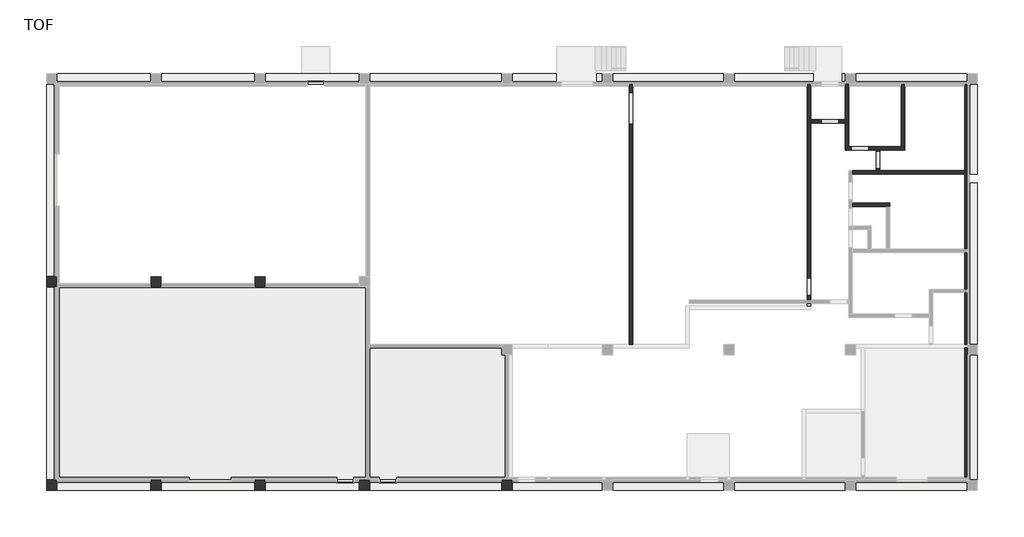
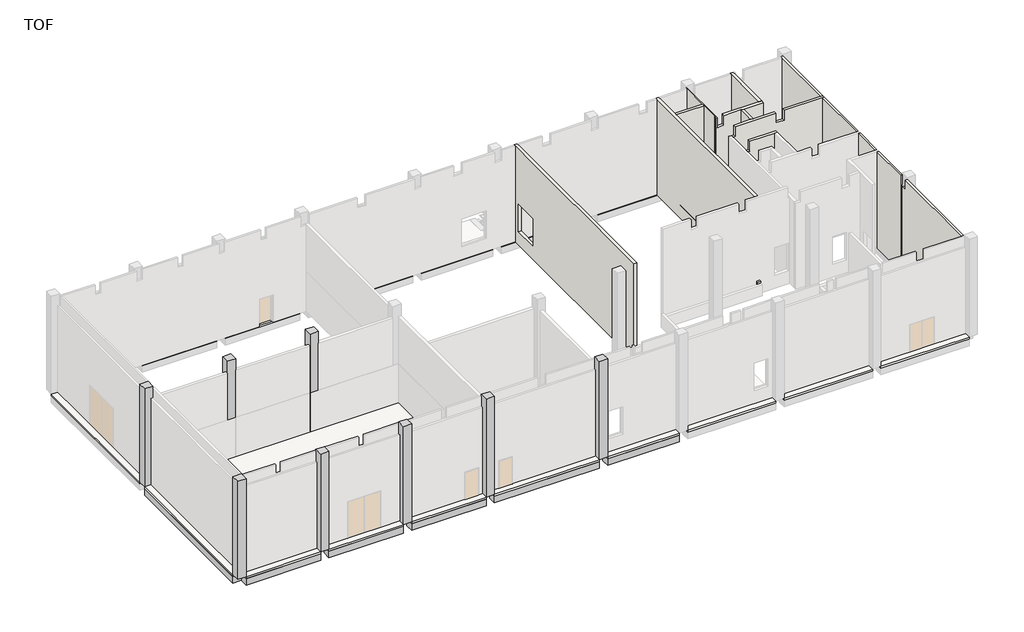
# One storey, part 3 of 4: 11 walls, 8 columns, 6 beams, 3 slabs, 1 proxy.
"""IFC4 building model written with IfcOpenShell, lengths in millimetres."""

from ifc_helpers import new_model, si_unit, frame, origin, place, context, project, spatial, polyline, outline, extrude, faceted_brep, element, save

model = new_model("IFC4")

# Units and contexts
model_context = context("Model", 3, world=origin())
ifc_project = project(units=[si_unit("LENGTHUNIT", "METRE", prefix="MILLI")], contexts=[model_context])

# Site, building, storey
site = spatial("IfcSite", under=ifc_project)
building = spatial("IfcBuilding", under=site)
storey = spatial("IfcBuildingStorey", under=building, Name="TOF", Elevation=149.9618634)

# Beams
placement = place(None, origin())
element("IfcBeam", 1, ObjectType="RC Beam_Rectangular : H_SB_AR_S16_TG_B600xH650_TG1", at=placement, inside=storey, context=model_context, shape_type="SweptSolid", body=[
    extrude(outline(polyline([(-300.0, 11899.5208589), (300.0, 11899.5208589), (300.0, 799.5208589), (-300.0, 799.5208589), (-300.0, 11899.5208589)])), frame((0.0, 0.0, -500.0381366), z_axis=(0.0, 0.0, 1.0), x_axis=(1.0, 0.0, 0.0)), (0.0, 0.0, 1.0), 500.0),
])
element("IfcBeam", 2, ObjectType="RC Beam_Rectangular : H_SB_AR_S16_TG_B600xH650_TG2", at=placement, inside=storey, context=model_context, shape_type="SweptSolid", body=[
    extrude(outline(polyline([(300.0, 199.5208589), (300.0, 799.5208589), (5700.0, 799.5208589), (5700.0, 199.5208589), (300.0, 199.5208589)])), frame((0.0, 0.0, -500.0381366), z_axis=(0.0, 0.0, 1.0), x_axis=(1.0, 0.0, 0.0)), (0.0, 0.0, 1.0), 500.0),
])
element("IfcBeam", 3, ObjectType="RC Beam_Rectangular : H_SB_AR_S16_TG_B600xH650_TG2", at=placement, inside=storey, context=model_context, shape_type="SweptSolid", body=[
    extrude(outline(polyline([(6300.0, 199.5208589), (6300.0, 799.5208589), (11700.0, 799.5208589), (11700.0, 199.5208589), (6300.0, 199.5208589)])), frame((0.0, 0.0, -500.0381366), z_axis=(0.0, 0.0, 1.0), x_axis=(1.0, 0.0, 0.0)), (0.0, 0.0, 1.0), 500.0),
])
element("IfcBeam", 4, ObjectType="RC Beam_Rectangular : H_SB_AR_S16_TG_B600xH650_TG2", at=placement, inside=storey, context=model_context, shape_type="SweptSolid", body=[
    extrude(outline(polyline([(12300.0, 199.5208589), (12300.0, 799.5208589), (17700.0, 799.5208589), (17700.0, 199.5208589), (12300.0, 199.5208589)])), frame((0.0, 0.0, -500.0381366), z_axis=(0.0, 0.0, 1.0), x_axis=(1.0, 0.0, 0.0)), (0.0, 0.0, 1.0), 500.0),
])
element("IfcBeam", 5, ObjectType="RC Beam_Rectangular : H_SB_AR_S16_TG_B600xH650_TG2", at=placement, inside=storey, context=model_context, shape_type="SweptSolid", body=[
    extrude(outline(polyline([(18300.0, 199.5208589), (18300.0, 799.5208589), (25900.0, 799.5208589), (25900.0, 199.5208589), (18300.0, 199.5208589)])), frame((0.0, 0.0, -500.0381366), z_axis=(0.0, 0.0, 1.0), x_axis=(1.0, 0.0, 0.0)), (0.0, 0.0, 1.0), 500.0),
])
element("IfcBeam", 6, ObjectType="RC Beam_Rectangular : H_SB_AR_S16_TG_B600xH650_TG2", at=placement, inside=storey, context=model_context, shape_type="SweptSolid", body=[
    extrude(outline(polyline([(26500.0, 199.5208589), (26500.0, 799.5208589), (31700.0, 799.5208589), (31700.0, 199.5208589), (26500.0, 199.5208589)])), frame((0.0, 0.0, -500.0381366), z_axis=(0.0, 0.0, 1.0), x_axis=(1.0, 0.0, 0.0)), (0.0, 0.0, 1.0), 500.0),
])

# Proxy
element("IfcBuildingElementProxy", 7, Name="H_SF_AR_B08_Stoop_T200", ObjectType="H_SF_AR_B08_Stoop_T200", at=placement, inside=storey, context=model_context, shape_type="Brep", body=[
    faceted_brep([(16000.0, 25749.5208589, -50.0381366), (16000.0, 25749.5208589, -350.0381366), (14400.0, 25749.5208589, -350.0381366), (14400.0, 25749.5208589, -50.0381366), (15400.0, 25149.5208589, -50.0381366), (15000.0, 25149.5208589, -50.0381366), (15700.0, 25449.5208589, -350.0381366), (14700.0, 25449.5208589, -350.0381366), (14400.0, 24199.5208589, -350.0381366), (14700.0, 24199.5208589, -350.0381366), (15000.0, 24199.5208589, -50.0381366), (14400.0, 24199.5208589, -50.0381366), (16000.0, 24199.5208589, -350.0381366), (16000.0, 24199.5208589, -50.0381366), (15400.0, 24199.5208589, -50.0381366), (15700.0, 24199.5208589, -350.0381366)], [[[0, 1, 2, 3]], [[4, 0, 3, 5]], [[6, 4, 5, 7]], [[1, 6, 7, 2]], [[8, 9, 10, 11]], [[3, 2, 8, 11]], [[5, 3, 11, 10]], [[7, 5, 10, 9]], [[2, 7, 9, 8]], [[12, 13, 14, 15]], [[13, 12, 1, 0]], [[14, 13, 0, 4]], [[15, 14, 4, 6]], [[12, 15, 6, 1]]]),
])

# Columns
element("IfcColumn", 8, ObjectType="RC_Column_Rectangular : H_SC_AR_S15_W600xL600", at=placement, inside=storey, context=model_context, shape_type="Brep", body=[
    faceted_brep([(300.0, 12499.5208589, 149.9618634), (300.0, 12099.5208589, 149.9618634), (300.0, 11899.5208589, 149.9618634), (150.0, 11899.5208589, 149.9618634), (-300.0, 11899.5208589, 149.9618634), (-300.0, 12499.5208589, 149.9618634), (150.0, 12499.5208589, 149.9618634), (300.0, 12499.5208589, 7649.9618634), (300.0, 11899.5208589, 7649.9618634), (300.0, 11899.5208589, 7499.9618634), (300.0, 11899.5208589, 6749.9618634), (300.0, 12499.5208589, 6749.9618634), (300.0, 12499.5208589, 7499.9618634), (-300.0, 11899.5208589, 7649.9618634), (-300.0, 11899.5208589, 7499.9618634), (-300.0, 11899.5208589, 6749.9618634), (-300.0, 12499.5208589, 7649.9618634), (-300.0, 12499.5208589, 7499.9618634), (-300.0, 12499.5208589, 6749.9618634)], [[[0, 1, 2, 3, 4, 5, 6]], [[7, 8, 9, 10, 2, 1, 0, 11, 12]], [[8, 13, 14, 15, 4, 3, 2, 10, 9]], [[13, 16, 17, 18, 5, 4, 15, 14]], [[16, 7, 12, 11, 0, 6, 5, 18, 17]], [[7, 16, 13, 8]]]),
])
element("IfcColumn", 9, ObjectType="RC_Column_Rectangular : H_SC_AR_S15_W600xL600", at=placement, inside=storey, context=model_context, shape_type="Brep", body=[
    faceted_brep([(6300.0, 12499.5208589, 149.9618634), (6300.0, 12099.5208589, 149.9618634), (6300.0, 11899.5208589, 149.9618634), (5700.0, 11899.5208589, 149.9618634), (5700.0, 12099.5208589, 149.9618634), (5700.0, 12499.5208589, 149.9618634), (6300.0, 12499.5208589, 7649.9618634), (6300.0, 11899.5208589, 7649.9618634), (6300.0, 11899.5208589, 7499.9618634), (6300.0, 11899.5208589, 6749.9618634), (6300.0, 12499.5208589, 6749.9618634), (6300.0, 12499.5208589, 7499.9618634), (5700.0, 11899.5208589, 7649.9618634), (5700.0, 11899.5208589, 7499.9618634), (5700.0, 11899.5208589, 6749.9618634), (5700.0, 12499.5208589, 7649.9618634), (5700.0, 12499.5208589, 7499.9618634), (5700.0, 12499.5208589, 6749.9618634)], [[[0, 1, 2, 3, 4, 5]], [[6, 7, 8, 9, 2, 1, 0, 10, 11]], [[7, 12, 13, 14, 3, 2, 9, 8]], [[12, 15, 16, 17, 5, 4, 3, 14, 13]], [[15, 6, 11, 10, 0, 5, 17, 16]], [[6, 15, 12, 7]]]),
])
element("IfcColumn", 10, ObjectType="RC_Column_Rectangular : H_SC_AR_S15_W600xL600", at=placement, inside=storey, context=model_context, shape_type="Brep", body=[
    faceted_brep([(12300.0, 12499.5208589, 149.9618634), (12300.0, 12099.5208589, 149.9618634), (12300.0, 11899.5208589, 149.9618634), (11700.0, 11899.5208589, 149.9618634), (11700.0, 12099.5208589, 149.9618634), (11700.0, 12499.5208589, 149.9618634), (12300.0, 12499.5208589, 7649.9618634), (12300.0, 11899.5208589, 7649.9618634), (12300.0, 11899.5208589, 7499.9618634), (12300.0, 11899.5208589, 6749.9618634), (12300.0, 12499.5208589, 6749.9618634), (12300.0, 12499.5208589, 7499.9618634), (11700.0, 11899.5208589, 7649.9618634), (11700.0, 11899.5208589, 7499.9618634), (11700.0, 11899.5208589, 6749.9618634), (11700.0, 12499.5208589, 7649.9618634), (11700.0, 12499.5208589, 7499.9618634), (11700.0, 12499.5208589, 6749.9618634)], [[[0, 1, 2, 3, 4, 5]], [[6, 7, 8, 9, 2, 1, 0, 10, 11]], [[7, 12, 13, 14, 3, 2, 9, 8]], [[12, 15, 16, 17, 5, 4, 3, 14, 13]], [[15, 6, 11, 10, 0, 5, 17, 16]], [[6, 15, 12, 7]]]),
])
element("IfcColumn", 11, ObjectType="RC_Column_Rectangular : H_SC_AR_S15_W600xL600", at=placement, inside=storey, context=model_context, shape_type="Brep", body=[
    faceted_brep([(300.0, 799.5208589, 149.9618634), (300.0, 649.5208589, 149.9618634), (300.0, 199.5208589, 149.9618634), (-300.0, 199.5208589, 149.9618634), (-300.0, 799.5208589, 149.9618634), (150.0, 799.5208589, 149.9618634), (300.0, 799.5208589, 7649.9618634), (300.0, 199.5208589, 7649.9618634), (300.0, 199.5208589, 7499.9618634), (300.0, 199.5208589, 6749.9618634), (300.0, 799.5208589, 6749.9618634), (300.0, 799.5208589, 7499.9618634), (-150.0, 199.5208589, 7649.9618634), (-300.0, 199.5208589, 7649.9618634), (-300.0, 799.5208589, 7649.9618634), (-300.0, 799.5208589, 7499.9618634), (-300.0, 799.5208589, 6749.9618634)], [[[0, 1, 2, 3, 4, 5]], [[6, 7, 8, 9, 2, 1, 0, 10, 11]], [[7, 12, 13, 3, 2, 9, 8]], [[13, 14, 15, 16, 4, 3]], [[14, 6, 11, 10, 0, 5, 4, 16, 15]], [[6, 14, 13, 12, 7]]]),
])
element("IfcColumn", 12, ObjectType="RC_Column_Rectangular : H_SC_AR_S15_W600xL600", at=placement, inside=storey, context=model_context, shape_type="Brep", body=[
    faceted_brep([(6300.0, 799.5208589, 149.9618634), (6300.0, 649.5208589, 149.9618634), (6300.0, 199.5208589, 149.9618634), (5700.0, 199.5208589, 149.9618634), (5700.0, 649.5208589, 149.9618634), (5700.0, 799.5208589, 149.9618634), (6300.0, 799.5208589, 7649.9618634), (6300.0, 199.5208589, 7649.9618634), (6300.0, 199.5208589, 7499.9618634), (6300.0, 199.5208589, 6749.9618634), (6300.0, 799.5208589, 6749.9618634), (6300.0, 799.5208589, 7499.9618634), (5700.0, 199.5208589, 7649.9618634), (5700.0, 199.5208589, 7499.9618634), (5700.0, 199.5208589, 6749.9618634), (5700.0, 799.5208589, 7649.9618634), (5700.0, 799.5208589, 7499.9618634), (5700.0, 799.5208589, 6749.9618634)], [[[0, 1, 2, 3, 4, 5]], [[6, 7, 8, 9, 2, 1, 0, 10, 11]], [[7, 12, 13, 14, 3, 2, 9, 8]], [[12, 15, 16, 17, 5, 4, 3, 14, 13]], [[15, 6, 11, 10, 0, 5, 17, 16]], [[6, 15, 12, 7]]]),
])
element("IfcColumn", 13, ObjectType="RC_Column_Rectangular : H_SC_AR_S15_W600xL600", at=placement, inside=storey, context=model_context, shape_type="Brep", body=[
    faceted_brep([(12300.0, 799.5208589, 149.9618634), (12300.0, 649.5208589, 149.9618634), (12300.0, 199.5208589, 149.9618634), (11700.0, 199.5208589, 149.9618634), (11700.0, 649.5208589, 149.9618634), (11700.0, 799.5208589, 149.9618634), (12300.0, 799.5208589, 7649.9618634), (12300.0, 199.5208589, 7649.9618634), (12300.0, 199.5208589, 7499.9618634), (12300.0, 199.5208589, 6749.9618634), (12300.0, 799.5208589, 6749.9618634), (12300.0, 799.5208589, 7499.9618634), (11700.0, 199.5208589, 7649.9618634), (11700.0, 199.5208589, 7499.9618634), (11700.0, 199.5208589, 6749.9618634), (11700.0, 799.5208589, 7649.9618634), (11700.0, 799.5208589, 7499.9618634), (11700.0, 799.5208589, 6749.9618634)], [[[0, 1, 2, 3, 4, 5]], [[6, 7, 8, 9, 2, 1, 0, 10, 11]], [[7, 12, 13, 14, 3, 2, 9, 8]], [[12, 15, 16, 17, 5, 4, 3, 14, 13]], [[15, 6, 11, 10, 0, 5, 17, 16]], [[6, 15, 12, 7]]]),
])
element("IfcColumn", 14, ObjectType="RC_Column_Rectangular : H_SC_AR_S15_W600xL600", at=placement, inside=storey, context=model_context, shape_type="Brep", body=[
    faceted_brep([(18300.0, 799.5208589, 149.9618634), (18300.0, 649.5208589, 149.9618634), (18300.0, 199.5208589, 149.9618634), (17700.0, 199.5208589, 149.9618634), (17700.0, 649.5208589, 149.9618634), (17700.0, 799.5208589, 149.9618634), (18088.0, 799.5208589, 149.9618634), (18100.0, 799.5208589, 149.9618634), (18300.0, 799.5208589, 7649.9618634), (18300.0, 199.5208589, 7649.9618634), (18300.0, 199.5208589, 7499.9618634), (18300.0, 199.5208589, 6749.9618634), (18300.0, 799.5208589, 6749.9618634), (18300.0, 799.5208589, 7499.9618634), (17700.0, 199.5208589, 7649.9618634), (17700.0, 199.5208589, 7499.9618634), (17700.0, 199.5208589, 6749.9618634), (17700.0, 799.5208589, 7649.9618634), (17700.0, 799.5208589, 7499.9618634), (17700.0, 799.5208589, 6749.9618634)], [[[0, 1, 2, 3, 4, 5, 6, 7]], [[8, 9, 10, 11, 2, 1, 0, 12, 13]], [[9, 14, 15, 16, 3, 2, 11, 10]], [[14, 17, 18, 19, 5, 4, 3, 16, 15]], [[17, 8, 13, 12, 0, 7, 6, 5, 19, 18]], [[8, 17, 14, 9]]]),
])
element("IfcColumn", 15, ObjectType="RC_Column_Rectangular : H_SC_AR_S15_W600xL600", at=placement, inside=storey, context=model_context, shape_type="Brep", body=[
    faceted_brep([(26500.0, 799.5208589, 149.9618634), (26500.0, 649.5208589, 149.9618634), (26500.0, 199.5208589, 149.9618634), (25900.0, 199.5208589, 149.9618634), (25900.0, 649.5208589, 149.9618634), (25900.0, 799.5208589, 149.9618634), (26100.0, 799.5208589, 149.9618634), (26300.0, 799.5208589, 149.9618634), (26500.0, 799.5208589, 7649.9618634), (26500.0, 199.5208589, 7649.9618634), (26500.0, 199.5208589, 7499.9618634), (26500.0, 199.5208589, 6749.9618634), (26500.0, 799.5208589, 6749.9618634), (26500.0, 799.5208589, 7499.9618634), (25900.0, 199.5208589, 7649.9618634), (25900.0, 199.5208589, 7499.9618634), (25900.0, 199.5208589, 6749.9618634), (25900.0, 799.5208589, 7649.9618634), (25900.0, 799.5208589, 7499.9618634), (25900.0, 799.5208589, 6749.9618634)], [[[0, 1, 2, 3, 4, 5, 6, 7]], [[8, 9, 10, 11, 2, 1, 0, 12, 13]], [[9, 14, 15, 16, 3, 2, 11, 10]], [[14, 17, 18, 19, 5, 4, 3, 16, 15]], [[17, 8, 13, 12, 0, 7, 6, 5, 19, 18]], [[8, 17, 14, 9]]]),
])

# Slabs
element("IfcSlab", 16, ObjectType="H_FL_AR_S17_RC Slab T150_PERI", at=placement, inside=storey, context=model_context, shape_type="Brep", body=[
    faceted_brep([(52700.0, 23599.5208589, -0.0381366), (53300.0, 23599.5208589, -0.0381366), (53300.0, 18399.5208589, -0.0381366), (52700.0, 18399.5208589, -0.0381366), (46300.0, 23599.5208589, -0.0381366), (46300.0, 24199.5208589, -0.0381366), (52700.0, 24199.5208589, -0.0381366), (46300.0, 24199.5208589, 149.9618634), (46300.0, 23749.5208589, 149.9618634), (46300.0, 23599.5208589, 149.9618634), (52700.0, 23599.5208589, 149.9618634), (52700.0, 23749.5208589, 149.9618634), (52700.0, 24199.5208589, 149.9618634), (53300.0, 23599.5208589, 149.9618634), (52850.0, 23599.5208589, 149.9618634), (52700.0, 18399.5208589, 149.9618634), (53300.0, 18399.5208589, 149.9618634)], [[[0, 1, 2, 3]], [[4, 5, 6, 0]], [[7, 8, 9, 10, 11, 12]], [[13, 14, 10, 15, 16]], [[5, 7, 12, 6]], [[1, 13, 16, 2]], [[5, 4, 9, 8, 7]], [[0, 10, 14, 13, 1]], [[10, 0, 6, 12, 11]], [[3, 2, 16, 15]], [[0, 10, 9, 4]], [[10, 0, 3, 15]]]),
    faceted_brep([(53300.0, 8599.5208589, -0.0381366), (52700.0, 8599.5208589, -0.0381366), (52700.0, 17899.5208589, -0.0381366), (53300.0, 17899.5208589, -0.0381366), (52700.0, 8599.5208589, 149.9618634), (52850.0, 8599.5208589, 149.9618634), (53300.0, 8599.5208589, 149.9618634), (53300.0, 17899.5208589, 149.9618634), (52700.0, 17899.5208589, 149.9618634)], [[[0, 1, 2, 3]], [[4, 5, 6, 7, 8]], [[6, 0, 3, 7]], [[1, 0, 6, 5, 4]], [[3, 2, 8, 7]], [[1, 4, 8, 2]]]),
    faceted_brep([(52700.0, 7999.5208589, -0.0381366), (53300.0, 7999.5208589, -0.0381366), (53300.0, 799.5208589, -0.0381366), (52700.0, 799.5208589, -0.0381366), (46300.0, 199.5208589, -0.0381366), (46300.0, 799.5208589, -0.0381366), (52700.0, 199.5208589, -0.0381366), (46300.0, 799.5208589, 149.9618634), (46300.0, 649.5208589, 149.9618634), (46300.0, 199.5208589, 149.9618634), (52700.0, 199.5208589, 149.9618634), (52700.0, 649.5208589, 149.9618634), (52700.0, 799.5208589, 149.9618634), (50425.0, 799.5208589, 149.9618634), (48625.0, 799.5208589, 149.9618634), (53300.0, 7999.5208589, 149.9618634), (52850.0, 7999.5208589, 149.9618634), (52700.0, 7999.5208589, 149.9618634), (52850.0, 799.5208589, 149.9618634), (53300.0, 799.5208589, 149.9618634)], [[[0, 1, 2, 3]], [[4, 5, 3, 6]], [[7, 8, 9, 10, 11, 12, 13, 14]], [[15, 16, 17, 12, 18, 19]], [[9, 4, 6, 10]], [[1, 15, 19, 2]], [[1, 0, 17, 16, 15]], [[5, 4, 9, 8, 7]], [[3, 12, 11, 10, 6]], [[12, 3, 2, 19, 18]], [[12, 3, 5, 7, 14, 13]], [[3, 12, 17, 0]]]),
    faceted_brep([(300.0, 12499.5208589, -0.0381366), (-300.0, 12499.5208589, -0.0381366), (-300.0, 23599.5208589, -0.0381366), (300.0, 23599.5208589, -0.0381366), (300.0, 24199.5208589, -0.0381366), (5700.0, 24199.5208589, -0.0381366), (5700.0, 23599.5208589, -0.0381366), (300.0, 24199.5208589, 149.9618634), (300.0, 23749.5208589, 149.9618634), (300.0, 23599.5208589, 149.9618634), (5700.0, 23599.5208589, 149.9618634), (5700.0, 23749.5208589, 149.9618634), (5700.0, 24199.5208589, 149.9618634), (-300.0, 12499.5208589, 149.9618634), (150.0, 12499.5208589, 149.9618634), (300.0, 12499.5208589, 149.9618634), (300.0, 16574.5208589, 149.9618634), (300.0, 19574.5208589, 149.9618634), (150.0, 23599.5208589, 149.9618634), (-300.0, 23599.5208589, 149.9618634)], [[[0, 1, 2, 3]], [[3, 4, 5, 6]], [[7, 8, 9, 10, 11, 12]], [[13, 14, 15, 16, 17, 9, 18, 19]], [[1, 13, 19, 2]], [[4, 7, 12, 5]], [[1, 0, 15, 14, 13]], [[3, 9, 8, 7, 4]], [[9, 3, 2, 19, 18]], [[6, 5, 12, 11, 10]], [[9, 3, 6, 10]], [[3, 9, 17, 16, 15, 0]]]),
    faceted_brep([(-300.0, 11899.5208589, -0.0381366), (300.0, 11899.5208589, -0.0381366), (300.0, 799.5208589, -0.0381366), (-300.0, 799.5208589, -0.0381366), (300.0, 199.5208589, -0.0381366), (5700.0, 799.5208589, -0.0381366), (5700.0, 199.5208589, -0.0381366), (300.0, 11899.5208589, 149.9618634), (150.0, 11899.5208589, 149.9618634), (-300.0, 11899.5208589, 149.9618634), (-300.0, 799.5208589, 149.9618634), (150.0, 799.5208589, 149.9618634), (300.0, 799.5208589, 149.9618634), (300.0, 649.5208589, 149.9618634), (300.0, 199.5208589, 149.9618634), (5700.0, 199.5208589, 149.9618634), (5700.0, 649.5208589, 149.9618634), (5700.0, 799.5208589, 149.9618634)], [[[0, 1, 2, 3]], [[4, 2, 5, 6]], [[7, 8, 9, 10, 11, 12]], [[12, 13, 14, 15, 16, 17]], [[14, 4, 6, 15]], [[9, 0, 3, 10]], [[1, 0, 9, 8, 7]], [[12, 2, 4, 14, 13]], [[2, 12, 11, 10, 3]], [[6, 5, 17, 16, 15]], [[12, 2, 1, 7]], [[2, 12, 17, 5]]]),
    faceted_brep([(6300.0, 23599.5208589, -0.0381366), (6300.0, 24199.5208589, -0.0381366), (11700.0, 24199.5208589, -0.0381366), (11700.0, 23599.5208589, -0.0381366), (6300.0, 24199.5208589, 149.9618634), (6300.0, 23749.5208589, 149.9618634), (6300.0, 23599.5208589, 149.9618634), (11700.0, 23599.5208589, 149.9618634), (11700.0, 23749.5208589, 149.9618634), (11700.0, 24199.5208589, 149.9618634)], [[[0, 1, 2, 3]], [[4, 5, 6, 7, 8, 9]], [[1, 4, 9, 2]], [[1, 0, 6, 5, 4]], [[3, 2, 9, 8, 7]], [[6, 0, 3, 7]]]),
    faceted_brep([(12300.0, 23599.5208589, -0.0381366), (12300.0, 24199.5208589, -0.0381366), (17700.0, 24199.5208589, -0.0381366), (17700.0, 23599.5208589, -0.0381366), (12300.0, 24199.5208589, 149.9618634), (12300.0, 23749.5208589, 149.9618634), (12300.0, 23599.5208589, 149.9618634), (14700.0, 23599.5208589, 149.9618634), (15700.0, 23599.5208589, 149.9618634), (17700.0, 23599.5208589, 149.9618634), (17700.0, 23749.5208589, 149.9618634), (17700.0, 24199.5208589, 149.9618634)], [[[0, 1, 2, 3]], [[4, 5, 6, 7, 8, 9, 10, 11]], [[1, 4, 11, 2]], [[1, 0, 6, 5, 4]], [[3, 2, 11, 10, 9]], [[6, 0, 3, 9, 8, 7]]]),
    faceted_brep([(18300.0, 23599.5208589, -0.0381366), (18300.0, 24199.5208589, -0.0381366), (25900.0, 24199.5208589, -0.0381366), (25900.0, 23599.5208589, -0.0381366), (18300.0, 24199.5208589, 149.9618634), (18300.0, 23749.5208589, 149.9618634), (18300.0, 23599.5208589, 149.9618634), (25900.0, 23599.5208589, 149.9618634), (25900.0, 23749.5208589, 149.9618634), (25900.0, 24199.5208589, 149.9618634)], [[[0, 1, 2, 3]], [[4, 5, 6, 7, 8, 9]], [[1, 4, 9, 2]], [[1, 0, 6, 5, 4]], [[3, 2, 9, 8, 7]], [[6, 0, 3, 7]]]),
    faceted_brep([(26500.0, 23599.5208589, -0.0381366), (26500.0, 24199.5208589, -0.0381366), (31700.0, 24199.5208589, -0.0381366), (31700.0, 23599.5208589, -0.0381366), (26500.0, 24199.5208589, 149.9618634), (26500.0, 23749.5208589, 149.9618634), (26500.0, 23599.5208589, 149.9618634), (31700.0, 23599.5208589, 149.9618634), (31700.0, 23749.5208589, 149.9618634), (31700.0, 24199.5208589, 149.9618634)], [[[0, 1, 2, 3]], [[4, 5, 6, 7, 8, 9]], [[1, 4, 9, 2]], [[1, 0, 6, 5, 4]], [[3, 2, 9, 8, 7]], [[6, 0, 3, 7]]]),
    faceted_brep([(32300.0, 23599.5208589, -0.0381366), (32300.0, 24199.5208589, -0.0381366), (38700.0, 24199.5208589, -0.0381366), (38700.0, 23599.5208589, -0.0381366), (32300.0, 24199.5208589, 149.9618634), (32300.0, 23749.5208589, 149.9618634), (32300.0, 23599.5208589, 149.9618634), (38700.0, 23599.5208589, 149.9618634), (38700.0, 23749.5208589, 149.9618634), (38700.0, 24199.5208589, 149.9618634)], [[[0, 1, 2, 3]], [[4, 5, 6, 7, 8, 9]], [[1, 4, 9, 2]], [[1, 0, 6, 5, 4]], [[3, 2, 9, 8, 7]], [[6, 0, 3, 7]]]),
    faceted_brep([(39300.0, 23599.5208589, -0.0381366), (39300.0, 24199.5208589, -0.0381366), (45700.0, 24199.5208589, -0.0381366), (45700.0, 23599.5208589, -0.0381366), (39300.0, 24199.5208589, 149.9618634), (39300.0, 23749.5208589, 149.9618634), (39300.0, 23599.5208589, 149.9618634), (45700.0, 23599.5208589, 149.9618634), (45700.0, 23749.5208589, 149.9618634), (45700.0, 24199.5208589, 149.9618634)], [[[0, 1, 2, 3]], [[4, 5, 6, 7, 8, 9]], [[1, 4, 9, 2]], [[1, 0, 6, 5, 4]], [[3, 2, 9, 8, 7]], [[6, 0, 3, 7]]]),
    faceted_brep([(6300.0, 199.5208589, -0.0381366), (6300.0, 799.5208589, -0.0381366), (11700.0, 799.5208589, -0.0381366), (11700.0, 199.5208589, -0.0381366), (6300.0, 799.5208589, 149.9618634), (6300.0, 649.5208589, 149.9618634), (6300.0, 199.5208589, 149.9618634), (11700.0, 199.5208589, 149.9618634), (11700.0, 649.5208589, 149.9618634), (11700.0, 799.5208589, 149.9618634), (10325.0, 799.5208589, 149.9618634), (7925.0, 799.5208589, 149.9618634)], [[[0, 1, 2, 3]], [[4, 5, 6, 7, 8, 9, 10, 11]], [[6, 0, 3, 7]], [[1, 0, 6, 5, 4]], [[3, 2, 9, 8, 7]], [[1, 4, 11, 10, 9, 2]]]),
    faceted_brep([(12300.0, 199.5208589, -0.0381366), (12300.0, 799.5208589, -0.0381366), (17700.0, 799.5208589, -0.0381366), (17700.0, 199.5208589, -0.0381366), (12300.0, 799.5208589, 149.9618634), (12300.0, 649.5208589, 149.9618634), (12300.0, 199.5208589, 149.9618634), (17700.0, 199.5208589, 149.9618634), (17700.0, 649.5208589, 149.9618634), (17700.0, 799.5208589, 149.9618634), (17400.0, 799.5208589, 149.9618634), (16400.0, 799.5208589, 149.9618634)], [[[0, 1, 2, 3]], [[4, 5, 6, 7, 8, 9, 10, 11]], [[6, 0, 3, 7]], [[1, 0, 6, 5, 4]], [[3, 2, 9, 8, 7]], [[1, 4, 11, 10, 9, 2]]]),
    faceted_brep([(18300.0, 199.5208589, -0.0381366), (18300.0, 799.5208589, -0.0381366), (25900.0, 799.5208589, -0.0381366), (25900.0, 199.5208589, -0.0381366), (18300.0, 799.5208589, 149.9618634), (18300.0, 649.5208589, 149.9618634), (18300.0, 199.5208589, 149.9618634), (25900.0, 199.5208589, 149.9618634), (25900.0, 649.5208589, 149.9618634), (25900.0, 799.5208589, 149.9618634), (19850.0, 799.5208589, 149.9618634), (18850.0, 799.5208589, 149.9618634)], [[[0, 1, 2, 3]], [[4, 5, 6, 7, 8, 9, 10, 11]], [[6, 0, 3, 7]], [[1, 0, 6, 5, 4]], [[3, 2, 9, 8, 7]], [[1, 4, 11, 10, 9, 2]]]),
    faceted_brep([(26500.0, 199.5208589, -0.0381366), (26500.0, 799.5208589, -0.0381366), (31700.0, 799.5208589, -0.0381366), (31700.0, 199.5208589, -0.0381366), (26500.0, 799.5208589, 149.9618634), (26500.0, 649.5208589, 149.9618634), (26500.0, 199.5208589, 149.9618634), (31700.0, 199.5208589, 149.9618634), (31700.0, 649.5208589, 149.9618634), (31700.0, 799.5208589, 149.9618634)], [[[0, 1, 2, 3]], [[4, 5, 6, 7, 8, 9]], [[6, 0, 3, 7]], [[1, 0, 6, 5, 4]], [[3, 2, 9, 8, 7]], [[1, 4, 9, 2]]]),
    faceted_brep([(32300.0, 199.5208589, -0.0381366), (32300.0, 799.5208589, -0.0381366), (38700.0, 799.5208589, -0.0381366), (38700.0, 199.5208589, -0.0381366), (32300.0, 799.5208589, 149.9618634), (32300.0, 649.5208589, 149.9618634), (32300.0, 199.5208589, 149.9618634), (38700.0, 199.5208589, 149.9618634), (38700.0, 649.5208589, 149.9618634), (38700.0, 799.5208589, 149.9618634)], [[[0, 1, 2, 3]], [[4, 5, 6, 7, 8, 9]], [[6, 0, 3, 7]], [[1, 0, 6, 5, 4]], [[3, 2, 9, 8, 7]], [[1, 4, 9, 2]]]),
    faceted_brep([(39300.0, 199.5208589, -0.0381366), (39300.0, 799.5208589, -0.0381366), (45700.0, 799.5208589, -0.0381366), (45700.0, 199.5208589, -0.0381366), (39300.0, 799.5208589, 149.9618634), (39300.0, 649.5208589, 149.9618634), (39300.0, 199.5208589, 149.9618634), (45700.0, 199.5208589, 149.9618634), (45700.0, 649.5208589, 149.9618634), (45700.0, 799.5208589, 149.9618634)], [[[0, 1, 2, 3]], [[4, 5, 6, 7, 8, 9]], [[6, 0, 3, 7]], [[1, 0, 6, 5, 4]], [[3, 2, 9, 8, 7]], [[1, 4, 9, 2]]]),
])
element("IfcSlab", 17, ObjectType="H_SF_AR_S17_SOG T150_GS1", at=placement, inside=storey, context=model_context, shape_type="Brep", body=[
    faceted_brep([(300.0, 11899.5208589, -0.0381366), (18200.0, 11899.5208589, -0.0381366), (18200.0, 8399.5208589, -0.0381366), (18200.0, 799.5208589, -0.0381366), (300.0, 799.5208589, -0.0381366), (300.0, 11899.5208589, 149.9618634), (300.0, 799.5208589, 149.9618634), (18200.0, 799.5208589, 149.9618634), (18200.0, 8399.5208589, 149.9618634), (18200.0, 11899.5208589, 149.9618634)], [[[0, 1, 2, 3, 4]], [[5, 6, 7, 8, 9]], [[1, 0, 5, 9]], [[3, 2, 1, 9, 8, 7]], [[4, 3, 7, 6]], [[0, 4, 6, 5]]]),
])
element("IfcSlab", 18, ObjectType="H_SF_AR_S17_SOG T150_GS1", at=placement, inside=storey, context=model_context, shape_type="SweptSolid", body=[
    extrude(outline(polyline([(18200.0, 8399.5208589), (26500.0, 8399.5208589), (26500.0, 799.5208589), (18200.0, 799.5208589), (18200.0, 8399.5208589)])), frame((0.0, 0.0, -0.0381366), z_axis=(0.0, 0.0, 1.0), x_axis=(1.0, 0.0, 0.0)), (0.0, 0.0, 1.0), 150.0),
])

# Walls
element("IfcWall", 19, ObjectType="H_WA_AR_B02_Int Wall_Block T200", at=placement, inside=storey, context=model_context, shape_type="Brep", body=[
    faceted_brep([(33250.0, 23599.5208589, 149.9618634), (33250.0, 23473.5208589, 149.9618634), (33250.0, 8599.5208589, 149.9618634), (33250.0, 8599.5208589, 7499.9618634), (33250.0, 23473.5208589, 7499.9618634), (33250.0, 23599.5208589, 7499.9618634), (33250.0, 23099.5208589, 1149.9618634), (33250.0, 23099.5208589, 3249.9618634), (33250.0, 21299.5208589, 3249.9618634), (33250.0, 21299.5208589, 1149.9618634), (33450.0, 8599.5208589, 149.9618634), (33450.0, 23473.5208589, 149.9618634), (33450.0, 23599.5208589, 149.9618634), (33450.0, 23599.5208589, 7499.9618634), (33450.0, 23473.5208589, 7499.9618634), (33450.0, 8599.5208589, 7499.9618634), (33450.0, 23099.5208589, 3249.9618634), (33450.0, 23099.5208589, 1149.9618634), (33450.0, 21299.5208589, 1149.9618634), (33450.0, 21299.5208589, 3249.9618634)], [[[0, 1, 2, 3, 4, 5], [6, 7, 8, 9]], [[10, 11, 12, 13, 14, 15], [16, 17, 18, 19]], [[2, 1, 0, 12, 11, 10]], [[12, 0, 5, 13]], [[7, 6, 17, 16]], [[8, 7, 16, 19]], [[9, 8, 19, 18]], [[6, 9, 18, 17]], [[5, 4, 3, 15, 14, 13]], [[2, 10, 15, 3]]]),
])
element("IfcWall", 20, ObjectType="H_WA_AR_B02_Int Wall_Block T200", at=placement, inside=storey, context=model_context, shape_type="Brep", body=[
    faceted_brep([(43700.0, 11149.5208589, 149.9618634), (43700.0, 21349.5208589, 149.9618634), (43700.0, 21549.5208589, 149.9618634), (43700.0, 23473.5208589, 149.9618634), (43700.0, 23599.5208589, 149.9618634), (43700.0, 23599.5208589, 7499.9618634), (43700.0, 23473.5208589, 7499.9618634), (43700.0, 21549.5208589, 7499.9618634), (43700.0, 21349.5208589, 7499.9618634), (43700.0, 11149.5208589, 7499.9618634), (43700.0, 12424.5208589, 3249.9618634), (43700.0, 12424.5208589, 1149.9618634), (43700.0, 11424.5208589, 1149.9618634), (43700.0, 11424.5208589, 3249.9618634), (43500.0, 23599.5208589, 149.9618634), (43500.0, 23473.5208589, 149.9618634), (43500.0, 11149.5208589, 149.9618634), (43500.0, 11149.5208589, 7499.9618634), (43500.0, 23473.5208589, 7499.9618634), (43500.0, 23599.5208589, 7499.9618634), (43500.0, 12424.5208589, 1149.9618634), (43500.0, 12424.5208589, 3249.9618634), (43500.0, 11424.5208589, 3249.9618634), (43500.0, 11424.5208589, 1149.9618634)], [[[0, 1, 2, 3, 4, 5, 6, 7, 8, 9], [10, 11, 12, 13]], [[14, 15, 16, 17, 18, 19], [20, 21, 22, 23]], [[4, 3, 2, 1, 0, 16, 15, 14]], [[4, 14, 19, 5]], [[16, 0, 9, 17]], [[21, 20, 11, 10]], [[22, 21, 10, 13]], [[23, 22, 13, 12]], [[20, 23, 12, 11]], [[9, 8, 7, 6, 5, 19, 18, 17]]]),
])
element("IfcWall", 21, ObjectType="H_WA_AR_B02_Int Wall_Block T200", at=placement, inside=storey, context=model_context, shape_type="SweptSolid", body=[
    extrude(outline(polyline([(149.9618634, 43700.0), (149.9618634, 45700.0), (7499.9618634, 45700.0), (7499.9618634, 43700.0), (149.9618634, 43700.0)]), holes=[polyline([(1149.9618634, 44300.0), (3249.9618634, 44300.0), (3249.9618634, 45300.0), (1149.9618634, 45300.0), (1149.9618634, 44300.0)])]), frame((0.0, 21349.5208589, 0.0), z_axis=(0.0, 1.0, 0.0), x_axis=(0.0, 0.0, 1.0)), (0.0, 0.0, 1.0), 200.0),
])
element("IfcWall", 22, ObjectType="H_WA_AR_B02_Int Wall_Block T200", at=placement, inside=storey, context=model_context, shape_type="Brep", body=[
    faceted_brep([(46095.0, 18399.5208589, 149.9618634), (52574.0, 18399.5208589, 149.9618634), (52700.0, 18399.5208589, 149.9618634), (52700.0, 18399.5208589, 7499.9618634), (52574.0, 18399.5208589, 7499.9618634), (49800.0, 18399.5208589, 7499.9618634), (49800.0, 18399.5208589, 6749.9618634), (49200.0, 18399.5208589, 6749.9618634), (49200.0, 18399.5208589, 7499.9618634), (46250.0, 18399.5208589, 7499.9618634), (46250.0, 18399.5208589, 6749.9618634), (46095.0, 18399.5208589, 6749.9618634), (52700.0, 18599.5208589, 149.9618634), (52574.0, 18599.5208589, 149.9618634), (47675.0, 18599.5208589, 149.9618634), (47475.0, 18599.5208589, 149.9618634), (46095.0, 18599.5208589, 149.9618634), (46095.0, 18599.5208589, 6749.9618634), (46250.0, 18599.5208589, 6749.9618634), (46250.0, 18599.5208589, 7499.9618634), (47475.0, 18599.5208589, 7499.9618634), (47675.0, 18599.5208589, 7499.9618634), (49200.0, 18599.5208589, 7499.9618634), (49200.0, 18599.5208589, 6749.9618634), (49800.0, 18599.5208589, 6749.9618634), (49800.0, 18599.5208589, 7499.9618634), (52574.0, 18599.5208589, 7499.9618634), (52700.0, 18599.5208589, 7499.9618634)], [[[0, 1, 2, 3, 4, 5, 6, 7, 8, 9, 10, 11]], [[12, 13, 14, 15, 16, 17, 18, 19, 20, 21, 22, 23, 24, 25, 26, 27]], [[2, 1, 0, 16, 15, 14, 13, 12]], [[2, 12, 27, 3]], [[16, 0, 11, 17]], [[18, 10, 9, 19]], [[10, 18, 17, 11]], [[7, 23, 22, 8]], [[23, 7, 6, 24]], [[24, 6, 5, 25]], [[9, 8, 22, 21, 20, 19]], [[5, 4, 3, 27, 26, 25]]]),
])
element("IfcWall", 23, ObjectType="H_WA_AR_B02_Int Wall_Block T200", at=placement, inside=storey, context=model_context, shape_type="Brep", body=[
    faceted_brep([(45700.0, 19799.5208589, 149.9618634), (47475.0, 19799.5208589, 149.9618634), (47675.0, 19799.5208589, 149.9618634), (49100.0, 19799.5208589, 149.9618634), (49100.0, 19799.5208589, 7499.9618634), (47675.0, 19799.5208589, 7499.9618634), (47475.0, 19799.5208589, 7499.9618634), (46250.0, 19799.5208589, 7499.9618634), (46250.0, 19799.5208589, 6749.9618634), (45750.0, 19799.5208589, 6749.9618634), (45750.0, 19799.5208589, 7499.9618634), (45700.0, 19799.5208589, 7499.9618634), (47045.0, 19799.5208589, 3249.9618634), (47045.0, 19799.5208589, 1149.9618634), (46045.0, 19799.5208589, 1149.9618634), (46045.0, 19799.5208589, 3249.9618634), (49100.0, 19999.5208589, 149.9618634), (48900.0, 19999.5208589, 149.9618634), (45900.0, 19999.5208589, 149.9618634), (45700.0, 19999.5208589, 149.9618634), (45700.0, 19999.5208589, 7499.9618634), (45750.0, 19999.5208589, 7499.9618634), (45750.0, 19999.5208589, 6749.9618634), (45900.0, 19999.5208589, 6749.9618634), (46250.0, 19999.5208589, 6749.9618634), (46250.0, 19999.5208589, 7499.9618634), (48900.0, 19999.5208589, 7499.9618634), (49100.0, 19999.5208589, 7499.9618634), (47045.0, 19999.5208589, 1149.9618634), (47045.0, 19999.5208589, 3249.9618634), (46045.0, 19999.5208589, 3249.9618634), (46045.0, 19999.5208589, 1149.9618634)], [[[0, 1, 2, 3, 4, 5, 6, 7, 8, 9, 10, 11], [12, 13, 14, 15]], [[16, 17, 18, 19, 20, 21, 22, 23, 24, 25, 26, 27], [28, 29, 30, 31]], [[3, 2, 1, 0, 19, 18, 17, 16]], [[3, 16, 27, 4]], [[19, 0, 11, 20]], [[29, 28, 13, 12]], [[30, 29, 12, 15]], [[31, 30, 15, 14]], [[28, 31, 14, 13]], [[24, 8, 7, 25]], [[8, 24, 23, 22, 9]], [[9, 22, 21, 10]], [[11, 10, 21, 20]], [[7, 6, 5, 4, 27, 26, 25]]]),
])
element("IfcWall", 24, ObjectType="H_WA_AR_B02_Int Wall_Block T200", at=placement, inside=storey, context=model_context, shape_type="Brep", body=[
    faceted_brep([(49100.0, 19999.5208589, 149.9618634), (49100.0, 23473.5208589, 149.9618634), (49100.0, 23599.5208589, 149.9618634), (49100.0, 23599.5208589, 7499.9618634), (49100.0, 23473.5208589, 7499.9618634), (49100.0, 19999.5208589, 7499.9618634), (48900.0, 23599.5208589, 149.9618634), (48900.0, 23473.5208589, 149.9618634), (48900.0, 19999.5208589, 149.9618634), (48900.0, 19999.5208589, 7499.9618634), (48900.0, 23473.5208589, 7499.9618634), (48900.0, 23599.5208589, 7499.9618634)], [[[0, 1, 2, 3, 4, 5]], [[6, 7, 8, 9, 10, 11]], [[2, 1, 0, 8, 7, 6]], [[2, 6, 11, 3]], [[8, 0, 5, 9]], [[5, 4, 3, 11, 10, 9]]]),
])
element("IfcWall", 25, ObjectType="H_WA_AR_B02_Int Wall_Block T200", at=placement, inside=storey, context=model_context, shape_type="SweptSolid", body=[
    extrude(outline(polyline([(19799.5208589, 149.9618634), (18599.5208589, 149.9618634), (18599.5208589, 7499.9618634), (19799.5208589, 7499.9618634), (19799.5208589, 149.9618634)]), holes=[polyline([(19724.5208589, 1149.9618634), (19724.5208589, 3249.9618634), (18724.5208589, 3249.9618634), (18724.5208589, 1149.9618634), (19724.5208589, 1149.9618634)])]), frame((47475.0, 0.0, 0.0), z_axis=(1.0, 0.0, 0.0), x_axis=(0.0, 1.0, 0.0)), (0.0, 0.0, 1.0), 200.0),
])
element("IfcWall", 26, ObjectType="H_WA_AR_B02_Int Wall_Block T200", at=placement, inside=storey, context=model_context, shape_type="Brep", body=[
    faceted_brep([(45900.0, 19999.5208589, 149.9618634), (45900.0, 23473.5208589, 149.9618634), (45900.0, 23599.5208589, 149.9618634), (45900.0, 23599.5208589, 6749.9618634), (45900.0, 23473.5208589, 6749.9618634), (45900.0, 19999.5208589, 6749.9618634), (45700.0, 23599.5208589, 149.9618634), (45700.0, 23473.5208589, 149.9618634), (45700.0, 21549.5208589, 149.9618634), (45700.0, 21349.5208589, 149.9618634), (45700.0, 19999.5208589, 149.9618634), (45700.0, 19999.5208589, 7499.9618634), (45700.0, 21349.5208589, 7499.9618634), (45700.0, 21549.5208589, 7499.9618634), (45700.0, 23473.5208589, 7499.9618634), (45700.0, 23599.5208589, 7499.9618634), (45750.0, 23599.5208589, 7499.9618634), (45750.0, 23599.5208589, 6749.9618634), (45750.0, 19999.5208589, 6749.9618634), (45750.0, 19999.5208589, 7499.9618634)], [[[0, 1, 2, 3, 4, 5]], [[6, 7, 8, 9, 10, 11, 12, 13, 14, 15]], [[2, 1, 0, 10, 9, 8, 7, 6]], [[2, 6, 15, 16, 17, 3]], [[10, 0, 5, 18, 19, 11]], [[17, 18, 5, 4, 3]], [[18, 17, 16, 19]], [[15, 14, 13, 12, 11, 19, 16]]]),
])
element("IfcWall", 27, ObjectType="H_WA_AR_B02_Int Wall_Block T200", at=placement, inside=storey, context=model_context, shape_type="Brep", body=[
    faceted_brep([(46095.0, 16549.5208589, 149.9618634), (48050.0, 16549.5208589, 149.9618634), (48250.0, 16549.5208589, 149.9618634), (48250.0, 16549.5208589, 7499.9618634), (48050.0, 16549.5208589, 7499.9618634), (46250.0, 16549.5208589, 7499.9618634), (46250.0, 16549.5208589, 6749.9618634), (46095.0, 16549.5208589, 6749.9618634), (48250.0, 16749.5208589, 149.9618634), (46095.0, 16749.5208589, 149.9618634), (46095.0, 16749.5208589, 6749.9618634), (46250.0, 16749.5208589, 6749.9618634), (46250.0, 16749.5208589, 7499.9618634), (48250.0, 16749.5208589, 7499.9618634)], [[[0, 1, 2, 3, 4, 5, 6, 7]], [[8, 9, 10, 11, 12, 13]], [[2, 1, 0, 9, 8]], [[9, 0, 7, 10]], [[2, 8, 13, 3]], [[11, 6, 5, 12]], [[6, 11, 10, 7]], [[5, 4, 3, 13, 12]]]),
])
element("IfcWall", 28, ObjectType="H_WA_AR_B02_Ext Wall_1L Gypsum_Mineral Wool_T110", at=placement, inside=storey, context=model_context, shape_type="Brep", body=[
    faceted_brep([(52574.0, 23599.5208589, 149.9618634), (52574.0, 23473.5208589, 149.9618634), (52574.0, 18599.5208589, 149.9618634), (52574.0, 18599.5208589, 7499.9618634), (52574.0, 23473.5208589, 7499.9618634), (52574.0, 23599.5208589, 7499.9618634), (52700.0, 18599.5208589, 149.9618634), (52700.0, 23599.5208589, 149.9618634), (52700.0, 23599.5208589, 6749.9618634), (52700.0, 23599.5208589, 7499.9618634), (52700.0, 18599.5208589, 7499.9618634)], [[[0, 1, 2, 3, 4, 5]], [[6, 7, 8, 9, 10]], [[0, 7, 6, 2, 1]], [[7, 0, 5, 9, 8]], [[2, 6, 10, 3]], [[5, 4, 3, 10, 9]]]),
    faceted_brep([(52574.0, 18399.5208589, 149.9618634), (52574.0, 14099.5208589, 149.9618634), (52574.0, 14099.5208589, 7499.9618634), (52574.0, 18399.5208589, 7499.9618634), (52700.0, 14099.5208589, 149.9618634), (52700.0, 18399.5208589, 149.9618634), (52700.0, 18399.5208589, 7499.9618634), (52700.0, 14099.5208589, 7499.9618634)], [[[0, 1, 2, 3]], [[4, 5, 6, 7]], [[0, 5, 4, 1]], [[5, 0, 3, 6]], [[1, 4, 7, 2]], [[3, 2, 7, 6]]]),
    faceted_brep([(52574.0, 11574.5208589, 149.9618634), (52574.0, 925.5208589, 149.9618634), (52574.0, 925.5208589, 7499.9618634), (52574.0, 7999.5208589, 7499.9618634), (52574.0, 7999.5208589, 6749.9618634), (52574.0, 8399.5208589, 6749.9618634), (52574.0, 8399.5208589, 1149.9618634), (52574.0, 8599.5208589, 1149.9618634), (52574.0, 8599.5208589, 7499.9618634), (52574.0, 11574.5208589, 7499.9618634), (52700.0, 925.5208589, 149.9618634), (52700.0, 7999.5208589, 149.9618634), (52700.0, 8599.5208589, 149.9618634), (52700.0, 11574.5208589, 149.9618634), (52700.0, 11574.5208589, 7499.9618634), (52700.0, 8599.5208589, 7499.9618634), (52700.0, 8599.5208589, 6749.9618634), (52700.0, 8599.5208589, 1149.9618634), (52700.0, 8399.5208589, 1149.9618634), (52700.0, 8399.5208589, 6749.9618634), (52700.0, 7999.5208589, 6749.9618634), (52700.0, 7999.5208589, 7499.9618634), (52700.0, 925.5208589, 7499.9618634)], [[[0, 1, 2, 3, 4, 5, 6, 7, 8, 9]], [[10, 11, 12, 13, 14, 15, 16, 17, 18, 19, 20, 21, 22]], [[10, 1, 0, 13, 12, 11]], [[1, 10, 22, 2]], [[13, 0, 9, 14]], [[18, 6, 5, 19]], [[6, 18, 17, 7]], [[20, 4, 3, 21]], [[4, 20, 19, 5]], [[7, 17, 16, 15, 8]], [[3, 2, 22, 21]], [[9, 8, 15, 14]]]),
    faceted_brep([(52574.0, 13899.5208589, 149.9618634), (52574.0, 11774.5208589, 149.9618634), (52574.0, 11774.5208589, 7499.9618634), (52574.0, 13899.5208589, 7499.9618634), (52700.0, 11774.5208589, 149.9618634), (52700.0, 13899.5208589, 149.9618634), (52700.0, 13899.5208589, 7499.9618634), (52700.0, 11774.5208589, 7499.9618634)], [[[0, 1, 2, 3]], [[4, 5, 6, 7]], [[0, 5, 4, 1]], [[5, 0, 3, 6]], [[1, 4, 7, 2]], [[3, 2, 7, 6]]]),
])
element("IfcWall", 29, ObjectType="H_WA_AR_B02_Int Wall_RC", at=placement, inside=storey, context=model_context, shape_type="Brep", body=[
    faceted_brep([(43700.0, 10799.5208589, 149.9618634), (43700.0, 23599.5208589, 149.9618634), (43700.0, 23599.5208589, 1149.9618634), (43700.0, 10799.5208589, 1149.9618634), (43700.0, 10799.5208589, 999.9618634), (43500.0, 10799.5208589, 149.9618634), (43500.0, 10799.5208589, 1149.9618634), (43500.0, 23599.5208589, 1149.9618634), (43500.0, 23599.5208589, 149.9618634)], [[[0, 1, 2, 3, 4]], [[5, 6, 7, 8]], [[1, 0, 5, 8]], [[3, 2, 7, 6]], [[2, 1, 8, 7]], [[0, 4, 3, 6, 5]]]),
])

save(model, "model.ifc")

# Revit data of these elements
# Type "RC Beam_Rectangular : H_SB_AR_S16_TG_B600xH650_TG1"
#   중앙부 하부근 = ""
#   중앙부 상부근 = ""
#   중앙부 보조근 = ""
#   중앙부 늑근 = ""
#   외단부 하부근 = ""
#   외단부 상부근 = ""
#   외단부 보조근 = ""
#   외단부 늑근 = ""
#   부호 = "TG2"
#   내단부 하부근 = ""
#   내단부 상부근 = ""
#   내단부 보조근 = ""
#   내단부 늑근 = ""
#   ALL 하부근 = "3-D20"
#   ALL 상부근 = "4-D20"
#   ALL 보조근 = ""
#   ALL 늑근 = "2-D10 @120"
#   Width = 600 mm
#   Height = 650 mm
#   Length [instance default] = 1524 mm
#   b = 600 mm
#   h = 650 mm
#   hec_material3 [instance default] = none
#   hec_material2 [instance default] = none
#   hec_material1 [instance default] = none
#   Structural Material [instance default] = none
#   Assembly Code = ""
# Type "RC Beam_Rectangular : H_SB_AR_S16_TG_B600xH650_TG2"
#   중앙부 하부근 = ""
#   중앙부 상부근 = ""
#   중앙부 보조근 = ""
#   중앙부 늑근 = ""
#   외단부 하부근 = ""
#   외단부 상부근 = ""
#   외단부 보조근 = ""
#   외단부 늑근 = ""
#   부호 = "TG2"
#   내단부 하부근 = ""
#   내단부 상부근 = ""
#   내단부 보조근 = ""
#   내단부 늑근 = ""
#   ALL 하부근 = "3-D20"
#   ALL 상부근 = "4-D20"
#   ALL 보조근 = ""
#   ALL 늑근 = "2-D10 @120"
#   Width = 600 mm
#   Height = 650 mm
#   Length [instance default] = 1524 mm
#   b = 600 mm
#   h = 650 mm
#   hec_material3 [instance default] = none
#   hec_material2 [instance default] = none
#   hec_material1 [instance default] = none
#   Structural Material [instance default] = none
#   Assembly Code = ""
# Type "RC_Column_Rectangular : H_SC_AR_S15_W600xL600"
#   Width = 600 mm
#   Length = 600 mm
#   hec_material3 [instance default] = none
#   hec_material2 [instance default] = none
#   hec_material1 [instance default] = none
#   Structural Material [instance default] = none
#   Description = (empty or 0)
# Type "H_FL_AR_S17_RC Slab T150_PERI"
#   Keynote = ""
#   Type Comments = ""
#   Description = ""
#   Function = 1
#   Layers, outside or top first: 150 mm "Concrete - Cast-in-Place Concrete - 35 MPa" (function 1)
# Type "H_SF_AR_S17_SOG T150_GS1"
#   Type Comments = "구조_콘크리트"
#   Layers, outside or top first: 150 mm "Concrete - Cast-in-Place Concrete - 35 MPa" (function 1)
# Type "H_WA_AR_B02_Int Wall_Block T200"
#   Type Comments = ""
#   Layers, outside or top first: 200 mm "00_Masonry_Conc. Block" (function 1)
# Type "H_WA_AR_B02_Ext Wall_1L Gypsum_Mineral Wool_T110"
#   Type Comments = "구조_콘크리트"
#   Layers, outside or top first: 110 mm "Rock Wool" (function 2); 16 mm "Gypsum Wall Board" (function 1)
# Type "H_WA_AR_B02_Int Wall_RC"
#   Type Comments = ""
#   Layers, outside or top first: 200 mm "Concrete - Cast-in-Place Concrete - 35 MPa" (function 1)
# Element 1 (IfcBeam, "RC Beam_Rectangular : H_SB_AR_S16_TG_B600xH650_TG1")
#   Comments = ""
#   hec_material3 = none
#   hec_material2 = none
#   hec_material1 = none
#   Structural Material = Concrete - Cast-in-Place Concrete - 35 MPa
#   Phase Created = New Construction
#   Materials on its faces: "Concrete - Cast-in-Place Concrete - 35 MPa"
# Elements 2, 3, 4, 5, 6 (IfcBeam, "RC Beam_Rectangular : H_SB_AR_S16_TG_B600xH650_TG2")
#   Comments = ""
#   hec_material3 = none
#   hec_material2 = none
#   hec_material1 = none
#   Structural Material = Concrete - Cast-in-Place Concrete - 35 MPa
#   Phase Created = New Construction
#   Materials on its faces: "Concrete - Cast-in-Place Concrete - 35 MPa"
# Element 7 (IfcBuildingElementProxy, "H_SF_AR_B08_Stoop_T200")
#   Phase Created = New Construction
#   Materials on its faces: "Concrete - Cast-in-Place Concrete - 35 MPa"
# Elements 8, 9, 10, 11, 12, 13, 14, 15 (IfcColumn, "RC_Column_Rectangular : H_SC_AR_S15_W600xL600")
#   Comments = ""
#   hec_material3 = none
#   hec_material2 = none
#   hec_material1 = none
#   Structural Material = Concrete - Cast-in-Place Concrete - 35 MPa
#   Phase Created = New Construction
#   Materials on its faces: "Concrete - Cast-in-Place Concrete - 35 MPa"
# Element 16 (IfcSlab, "H_FL_AR_S17_RC Slab T150_PERI")
#   Height Offset From Level = 0 mm
#   Phase Created = New Construction
#   Materials on its faces: "Concrete - Cast-in-Place Concrete - 35 MPa"
# Elements 17, 18 (IfcSlab, "H_SF_AR_S17_SOG T150_GS1")
#   Comments = ""
#   built-in parameter 1001955 = 1.5708 (stored number, unit not read)
#   Height Offset From Level = 0 mm
#   built-in parameter 1001954 = 1
#   Phase Created = New Construction
#   Materials on its faces: "Concrete - Cast-in-Place Concrete - 35 MPa"
# Elements 19, 20, 21, 22, 23, 24, 25, 26, 27 (IfcWall, "H_WA_AR_B02_Int Wall_Block T200")
#   H_Wall Style Name = "Block Wall"
#   H_Wall-Base Material-1 = "Concrete Block"
#   H_Wall-Base Material-2 = ""
#   H_Wall_Finish-In = "Acrylic Emulsion Paint on Cement Plaster"
#   H_Wall_Base Material-3 = ""
#   H_Wall_Finish-Ex = "Acrylic Emulsion Paint on Cement Plaster"
#   H_Wall_Style Remark = "WM : Reinforced Concrete Block\n     50mm<THK≤100mm / 100mm<THK≤200mm / 200mm<THK"
#   Top Offset = 0 mm
#   Base Offset = 0 mm
#   wall height = 7500 mm
#   H_Wall Style No = IW21
#   Phase Created = New Construction
#   Base Constraint = TOF
#   Top Constraint = TOC
#   Materials on its faces: "00_Masonry_Conc. Block"
# Element 28 (IfcWall, "H_WA_AR_B02_Ext Wall_1L Gypsum_Mineral Wool_T110")
#   Top Offset = 0 mm
#   Base Offset = 0 mm
#   wall height = 7500 mm
#   Phase Created = New Construction
#   Base Constraint = TOF
#   Top Constraint = TOC
#   Materials on its faces: "Rock Wool", "Gypsum Wall Board"
# Element 29 (IfcWall, "H_WA_AR_B02_Int Wall_RC")
#   Top Offset = 0 mm
#   Base Offset = 0 mm
#   wall height = 1000 mm
#   Phase Created = New Construction
#   Base Constraint = TOF
#   Top Constraint = TOF2
#   Materials on its faces: "Concrete - Cast-in-Place Concrete - 35 MPa"
# Materials
#   "Concrete - Cast-in-Place Concrete - 35 MPa": class "Concrete", colour RGB 192 192 192, transparency 0, Cost = 0
#   "00_Masonry_Conc. Block": class "Concrete", colour RGB 180 180 180, transparency 0, Description = "Conc. Block", Cost = 0, Image = Brick_Uniform_12inch_Running_Gray.png
#   "Rock Wool": class "Generic", colour RGB 120 120 120, transparency 0, Description = "Rock Wool", Cost = 0
#   "Gypsum Wall Board": class "Generic", colour RGB 171 170 168, transparency 0, Description = "Gypsum Wall Board", Cost = 0
